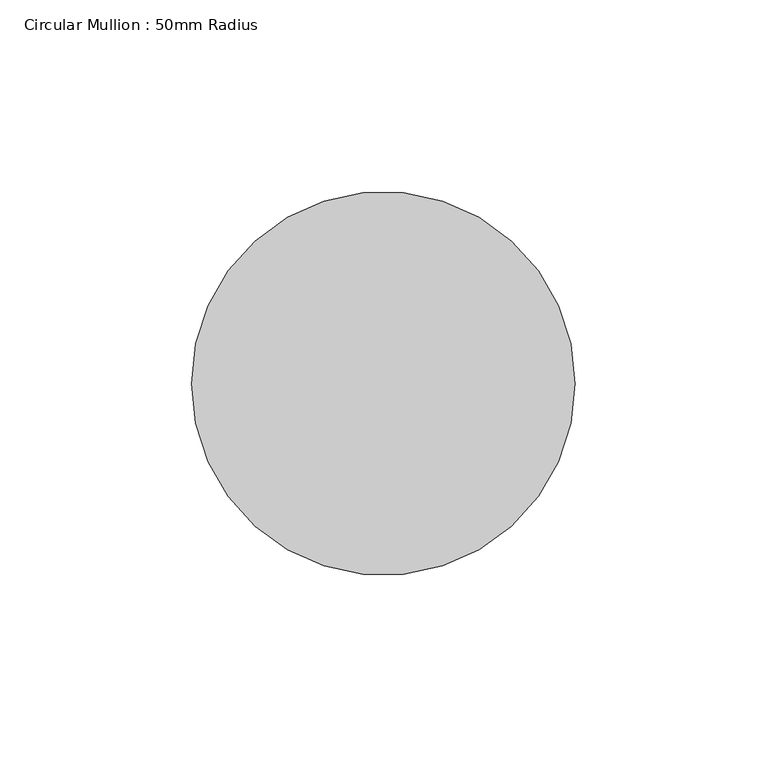
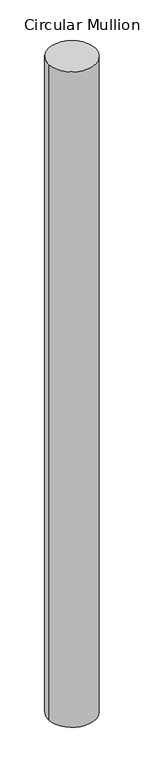
"""IFC4 building model written with IfcOpenShell, lengths in millimetres: member geometry, Circular Mullion : 50mm Radius."""

from ifc_helpers import new_model, si_unit, point, frame, origin, origin_2d, place, context, project, spatial, circle_curve, trimmed, segment, composite_curve, outline, extrude, source, transform, mapped, element, save


def circular_mullion_50mm_radius_46d4ac40(model_context):
    return source(origin(), model_context, "Body", "SweptSolid", [
        extrude(outline(composite_curve([segment(trimmed(circle_curve(origin_2d(), 50.0), [point((50.0, 0.0))], [point((-50.0, 0.0))], False, "CARTESIAN"), True, "CONTINUOUS"), segment(trimmed(circle_curve(origin_2d(), 50.0), [point((-50.0, 0.0))], [point((50.0, 0.0))], False, "CARTESIAN"), True, "CONTINUOUS")], self_intersect=False)), frame((0.0, 0.0, -1465.4436505), z_axis=(0.0, 0.0, 1.0), x_axis=(1.0, 0.0, 0.0)), (0.0, 0.0, 1.0), 1465.4436505),
    ])


if __name__ == "__main__":
    model = new_model("IFC4")
    model_context = context("Model", 3, world=origin())
    ifc_project = project(units=[si_unit("LENGTHUNIT", "METRE", prefix="MILLI")], contexts=[model_context])
    site = spatial("IfcSite", under=ifc_project)
    building = spatial("IfcBuilding", under=site)
    placement = place(None, origin())
    circular_mullion_50mm_radius_shape = circular_mullion_50mm_radius_46d4ac40(model_context)
    element("IfcMember", 1, ObjectType="Circular Mullion : 50mm Radius", at=placement, inside=building, context=model_context, shape_type="MappedRepresentation", body=[
        mapped(circular_mullion_50mm_radius_shape, transform((0.0, 0.0, 0.0), x_axis=(1.0, 0.0, 0.0), y_axis=(0.0, 1.0, 0.0), z_axis=(0.0, 0.0, 1.0))),
    ])
    save(model, "model.ifc")

# Revit data of these elements
# Type "Circular Mullion : 50mm Radius"
#   built-in parameter 1007350 = 0.164042 (stored number, unit not read)
# Element 1 (IfcMember, "Circular Mullion : 50mm Radius")
#   Materials on its faces: "Aluminium"
# Materials
#   "Aluminium": class "Metal", colour RGB 247 247 247, transparency 0, Description = "Aluminium 6061", Cost = 0
